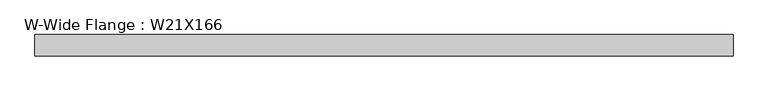
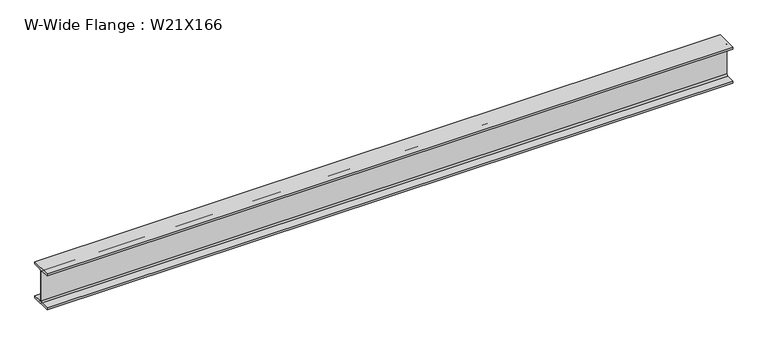
"""IFC4 building model written with IfcOpenShell, lengths in millimetres: beam geometry, W-Wide Flange : W21X166."""

from ifc_helpers import new_model, si_unit, point, frame, frame_2d, origin, place, context, project, spatial, polyline, circle_curve, trimmed, segment, composite_curve, outline, extrude, source, transform, mapped, element, save


def w_wide_flange_w21x166_41bf6792(model_context):
    return source(origin(), model_context, "Body", "SweptSolid", [
        extrude(outline(composite_curve([segment(polyline([(157.48, -251.206), (157.48, -285.75), (-157.48, -285.75), (-157.48, -251.206), (-32.131, -251.206)]), True, "CONTINUOUS"), segment(trimmed(circle_curve(frame_2d((-32.131, -228.6)), 22.606), [point((-32.131, -251.206))], [point((-9.525, -228.6))], True, "CARTESIAN"), True, "CONTINUOUS"), segment(polyline([(-9.525, -228.6), (-9.525, 228.6)]), True, "CONTINUOUS"), segment(trimmed(circle_curve(frame_2d((-32.131, 228.6)), 22.606), [point((-9.525, 228.6))], [point((-32.131, 251.206))], True, "CARTESIAN"), True, "CONTINUOUS"), segment(polyline([(-32.131, 251.206), (-157.48, 251.206), (-157.48, 285.75), (157.48, 285.75), (157.48, 251.206), (32.131, 251.206)]), True, "CONTINUOUS"), segment(trimmed(circle_curve(frame_2d((32.131, 228.6)), 22.606), [point((32.131, 251.206))], [point((9.525, 228.6))], True, "CARTESIAN"), True, "CONTINUOUS"), segment(polyline([(9.525, 228.6), (9.525, -228.6)]), True, "CONTINUOUS"), segment(trimmed(circle_curve(frame_2d((32.131, -228.6)), 22.606), [point((9.525, -228.6))], [point((32.131, -251.206))], True, "CARTESIAN"), True, "CONTINUOUS"), segment(polyline([(32.131, -251.206), (157.48, -251.206)]), True, "CONTINUOUS")], self_intersect=False)), frame((-5180.0235462, 0.0, 0.0), z_axis=(1.0, 0.0, 0.0), x_axis=(0.0, 1.0, 0.0)), (0.0, 0.0, 1.0), 10224.7221576),
    ])


if __name__ == "__main__":
    model = new_model("IFC4")
    model_context = context("Model", 3, world=origin())
    ifc_project = project(units=[si_unit("LENGTHUNIT", "METRE", prefix="MILLI")], contexts=[model_context])
    site = spatial("IfcSite", under=ifc_project)
    building = spatial("IfcBuilding", under=site)
    placement = place(None, origin())
    w_wide_flange_w21x166_shape = w_wide_flange_w21x166_41bf6792(model_context)
    element("IfcBeam", 1, ObjectType="W-Wide Flange : W21X166", at=placement, inside=building, context=model_context, shape_type="MappedRepresentation", body=[
        mapped(w_wide_flange_w21x166_shape, transform((0.0, 0.0, 0.0), x_axis=(1.0, 0.0, 0.0), y_axis=(0.0, 1.0, 0.0), z_axis=(0.0, 0.0, 1.0))),
    ])
    save(model, "model.ifc")

# Revit data of these elements
# Type "W-Wide Flange : W21X166"
#   Assembly Code = "B10"
#   W = 166
#   Length [instance default] = 5' - 0"
#   bf = 1' - 0.4"
#   d = 1' - 10 1/2"
#   k = 0' - 2 1/4"
#   k2 = 0' - 0.89"
#   tf = 0' - 1.36"
#   tw = 0' - 0 3/4"
#   A = 0.338889 SF
#   Structural Material [instance default] = Steel ASTM A992
# Element 1 (IfcBeam, "W-Wide Flange : W21X166")
#   Materials on its faces: "Steel ASTM A992"
# Materials
#   "Steel ASTM A992": class "Metal", colour RGB 199 199 199, transparency 0, Description = "Structural steel 50ksi", Cost = 0
